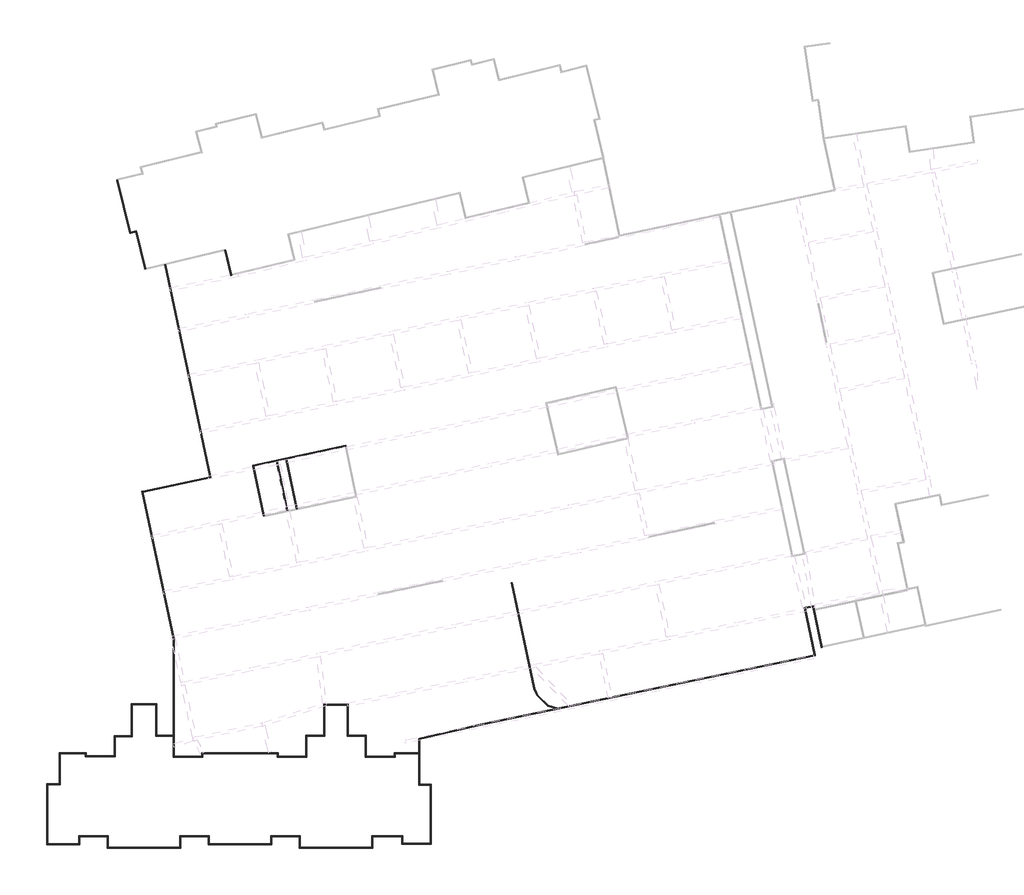
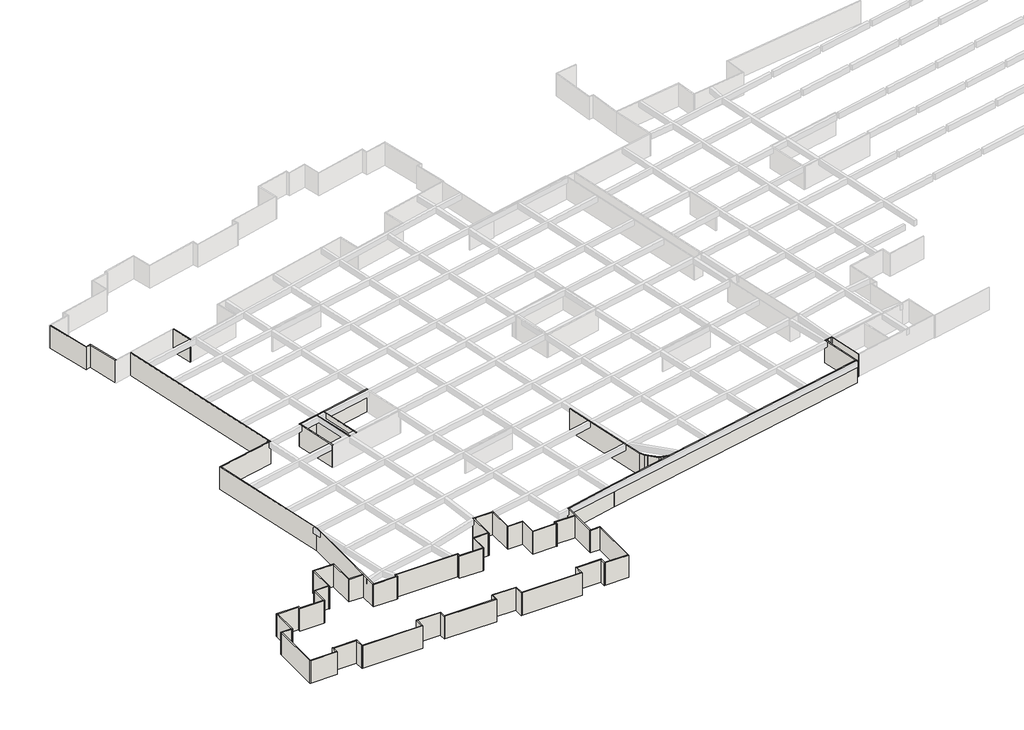
# One storey, part 1 of 14: 68 walls.
"""IFC4 building model written with IfcOpenShell, lengths in millimetres."""

from ifc_helpers import new_model, si_unit, origin, origin_with_axes, place, context, project, spatial, polyline, outline, extrude, faceted_brep, element, save

model = new_model("IFC4")

# Units and contexts
model_context = context("Model", 3, world=origin())
ifc_project = project(units=[si_unit("LENGTHUNIT", "METRE", prefix="MILLI")], contexts=[model_context])

# Site, building, storey
site = spatial("IfcSite", under=ifc_project)
building = spatial("IfcBuilding", under=site)
storey = spatial("IfcBuildingStorey", under=building, Name="户型图", Elevation=0.0)

# Walls
placement = place(None, origin())
element("IfcWall", 1, ObjectType="所有墙体", at=placement, inside=storey, context=model_context, shape_type="Brep", body=[
    faceted_brep([(-336633.0955644, -203222.3430669, 0.0), (-339553.0955247, -203222.3430669, 0.0), (-339553.0955247, -203222.3430669, 3300.0), (-336633.0955644, -203222.3430669, 3300.0), (-336633.0955644, -203342.3430669, 0.0), (-336633.0955644, -203342.3430669, 3300.0), (-336753.0955644, -203342.3430669, 3300.0), (-339433.0955247, -203342.3430669, 3300.0), (-339553.0955247, -203342.3430669, 3300.0), (-339553.0955247, -203342.3430669, 0.0), (-339433.0955247, -203342.3430669, 0.0), (-336753.0955644, -203342.3430669, 0.0)], [[[0, 1, 2, 3]], [[4, 5, 6, 7, 8, 9, 10, 11]], [[1, 0, 4, 11, 10, 9]], [[3, 2, 8, 7, 6, 5]], [[2, 1, 9, 8]], [[0, 3, 5, 4]]]),
])
element("IfcWall", 2, ObjectType="所有墙体", at=placement, inside=storey, context=model_context, shape_type="Brep", body=[
    faceted_brep([(-339553.0955247, -203342.3430669, 0.0), (-339553.0955247, -206922.3429831, 0.0), (-339553.0955247, -207042.3429831, 0.0), (-339553.0955247, -207042.3429831, 3300.0), (-339553.0955247, -206922.3429831, 3300.0), (-339553.0955247, -203342.3430669, 3300.0), (-339433.0955247, -203342.3430669, 0.0), (-339433.0955247, -203342.3430669, 3300.0), (-339433.0955247, -207042.3429831, 3300.0), (-339433.0955247, -207042.3429831, 0.0)], [[[0, 1, 2, 3, 4, 5]], [[6, 7, 8, 9]], [[2, 1, 0, 6, 9]], [[5, 4, 3, 8, 7]], [[0, 5, 7, 6]], [[3, 2, 9, 8]]]),
])
element("IfcWall", 3, ObjectType="所有墙体", at=placement, inside=storey, context=model_context, shape_type="Brep", body=[
    faceted_brep([(-339553.0955247, -206922.3429831, 0.0), (-341553.0955629, -206922.3429831, 0.0), (-341553.0955629, -206922.3429831, 3300.0), (-339553.0955247, -206922.3429831, 3300.0), (-339553.0955247, -207042.3429831, 0.0), (-339553.0955247, -207042.3429831, 3300.0), (-341433.0955629, -207042.3429831, 3300.0), (-341553.0955629, -207042.3429831, 3300.0), (-341553.0955629, -207042.3429831, 0.0), (-341433.0955629, -207042.3429831, 0.0)], [[[0, 1, 2, 3]], [[4, 5, 6, 7, 8, 9]], [[1, 0, 4, 9, 8]], [[3, 2, 7, 6, 5]], [[0, 3, 5, 4]], [[2, 1, 8, 7]]]),
])
element("IfcWall", 4, ObjectType="所有墙体", at=placement, inside=storey, context=model_context, shape_type="Brep", body=[
    faceted_brep([(-341553.0955629, -207042.3429831, 0.0), (-341553.0955629, -209222.3430662, 0.0), (-341553.0955629, -209342.3430662, 0.0), (-341553.0955629, -209342.3430662, 3300.0), (-341553.0955629, -209222.3430662, 3300.0), (-341553.0955629, -207042.3429831, 3300.0), (-341433.0955629, -207042.3429831, 0.0), (-341433.0955629, -207042.3429831, 3300.0), (-341433.0955629, -209342.3430662, 3300.0), (-341433.0955629, -209342.3430662, 0.0)], [[[0, 1, 2, 3, 4, 5]], [[6, 7, 8, 9]], [[2, 1, 0, 6, 9]], [[5, 4, 3, 8, 7]], [[0, 5, 7, 6]], [[3, 2, 9, 8]]]),
])
element("IfcWall", 5, ObjectType="所有墙体", at=placement, inside=storey, context=model_context, shape_type="Brep", body=[
    faceted_brep([(-341553.0955629, -209222.3430662, 0.0), (-344783.0955149, -209222.3430662, 0.0), (-344903.0955149, -209222.3430662, 0.0), (-344903.0955149, -209222.3430662, 3300.0), (-344783.0955149, -209222.3430662, 3300.0), (-341553.0955629, -209222.3430662, 3300.0), (-341553.0955629, -209342.3430662, 0.0), (-341553.0955629, -209342.3430662, 3300.0), (-344903.0955149, -209342.3430662, 3300.0), (-344903.0955149, -209342.3430662, 0.0)], [[[0, 1, 2, 3, 4, 5]], [[6, 7, 8, 9]], [[2, 1, 0, 6, 9]], [[5, 4, 3, 8, 7]], [[0, 5, 7, 6]], [[3, 2, 9, 8]]]),
])
element("IfcWall", 6, ObjectType="所有墙体", at=placement, inside=storey, context=model_context, shape_type="Brep", body=[
    faceted_brep([(-344783.0955149, -209222.3430662, 0.0), (-344783.0955149, -208872.3428754, 0.0), (-344783.0955149, -208872.3428754, 3300.0), (-344783.0955149, -209222.3430662, 3300.0), (-344903.0955149, -209222.3430662, 0.0), (-344903.0955149, -209222.3430662, 3300.0), (-344903.0955149, -208992.3428754, 3300.0), (-344903.0955149, -208872.3428754, 3300.0), (-344903.0955149, -208872.3428754, 0.0), (-344903.0955149, -208992.3428754, 0.0)], [[[0, 1, 2, 3]], [[4, 5, 6, 7, 8, 9]], [[1, 0, 4, 9, 8]], [[3, 2, 7, 6, 5]], [[0, 3, 5, 4]], [[2, 1, 8, 7]]]),
])
element("IfcWall", 7, ObjectType="所有墙体", at=placement, inside=storey, context=model_context, shape_type="Brep", body=[
    faceted_brep([(-344903.0955149, -208872.3428754, 0.0), (-347903.0955133, -208872.3428754, 0.0), (-347903.0955133, -208872.3428754, 3300.0), (-344903.0955149, -208872.3428754, 3300.0), (-344903.0955149, -208992.3428754, 0.0), (-344903.0955149, -208992.3428754, 3300.0), (-347783.0955133, -208992.3428754, 3300.0), (-347903.0955133, -208992.3428754, 3300.0), (-347903.0955133, -208992.3428754, 0.0), (-347783.0955133, -208992.3428754, 0.0)], [[[0, 1, 2, 3]], [[4, 5, 6, 7, 8, 9]], [[1, 0, 4, 9, 8]], [[3, 2, 7, 6, 5]], [[0, 3, 5, 4]], [[2, 1, 8, 7]]]),
])
element("IfcWall", 8, ObjectType="所有墙体", at=placement, inside=storey, context=model_context, shape_type="Brep", body=[
    faceted_brep([(-347903.0955133, -208992.3428754, 0.0), (-347903.0955133, -212472.3429639, 0.0), (-347903.0955133, -212592.3429639, 0.0), (-347903.0955133, -212592.3429639, 3300.0), (-347903.0955133, -212472.3429639, 3300.0), (-347903.0955133, -208992.3428754, 3300.0), (-347783.0955133, -208992.3428754, 0.0), (-347783.0955133, -208992.3428754, 3300.0), (-347783.0955133, -212592.3429639, 3300.0), (-347783.0955133, -212592.3429639, 0.0)], [[[0, 1, 2, 3, 4, 5]], [[6, 7, 8, 9]], [[2, 1, 0, 6, 9]], [[5, 4, 3, 8, 7]], [[0, 5, 7, 6]], [[3, 2, 9, 8]]]),
])
element("IfcWall", 9, ObjectType="所有墙体", at=placement, inside=storey, context=model_context, shape_type="Brep", body=[
    faceted_brep([(-347903.0955133, -212472.3429639, 0.0), (-349353.0955304, -212472.3429639, 0.0), (-349353.0955304, -212472.3429639, 3300.0), (-347903.0955133, -212472.3429639, 3300.0), (-347903.0955133, -212592.3429639, 0.0), (-347903.0955133, -212592.3429639, 3300.0), (-349233.0955304, -212592.3429639, 3300.0), (-349353.0955304, -212592.3429639, 3300.0), (-349353.0955304, -212592.3429639, 0.0), (-349233.0955304, -212592.3429639, 0.0)], [[[0, 1, 2, 3]], [[4, 5, 6, 7, 8, 9]], [[1, 0, 4, 9, 8]], [[3, 2, 7, 6, 5]], [[0, 3, 5, 4]], [[2, 1, 8, 7]]]),
])
element("IfcWall", 10, ObjectType="所有墙体", at=placement, inside=storey, context=model_context, shape_type="Brep", body=[
    faceted_brep([(-349353.0955304, -212592.3429639, 0.0), (-349353.0955304, -219492.3429639, 0.0), (-349353.0955304, -219492.3429639, 3300.0), (-349353.0955304, -212592.3429639, 3300.0), (-349233.0955304, -212592.3429639, 0.0), (-349233.0955304, -212592.3429639, 3300.0), (-349233.0955304, -219372.3429639, 3300.0), (-349233.0955304, -219492.3429639, 3300.0), (-349233.0955304, -219492.3429639, 0.0), (-349233.0955304, -219372.3429639, 0.0)], [[[0, 1, 2, 3]], [[4, 5, 6, 7, 8, 9]], [[1, 0, 4, 9, 8]], [[3, 2, 7, 6, 5]], [[0, 3, 5, 4]], [[2, 1, 8, 7]]]),
])
element("IfcWall", 11, ObjectType="所有墙体", at=placement, inside=storey, context=model_context, shape_type="Brep", body=[
    faceted_brep([(-349233.0955304, -219492.3429639, 0.0), (-345533.0955632, -219492.3429639, 0.0), (-345533.0955632, -219492.3429639, 3300.0), (-349233.0955304, -219492.3429639, 3300.0), (-349233.0955304, -219372.3429639, 0.0), (-349233.0955304, -219372.3429639, 3300.0), (-345653.0955632, -219372.3429639, 3300.0), (-345533.0955632, -219372.3429639, 3300.0), (-345533.0955632, -219372.3429639, 0.0), (-345653.0955632, -219372.3429639, 0.0)], [[[0, 1, 2, 3]], [[4, 5, 6, 7, 8, 9]], [[1, 0, 4, 9, 8]], [[3, 2, 7, 6, 5]], [[0, 3, 5, 4]], [[2, 1, 8, 7]]]),
])
element("IfcWall", 12, ObjectType="所有墙体", at=placement, inside=storey, context=model_context, shape_type="Brep", body=[
    faceted_brep([(-345533.0955632, -219372.3429639, 0.0), (-345533.0955632, -218592.3429692, 0.0), (-345533.0955632, -218472.3429692, 0.0), (-345533.0955632, -218472.3429692, 3300.0), (-345533.0955632, -218592.3429692, 3300.0), (-345533.0955632, -219372.3429639, 3300.0), (-345653.0955632, -219372.3429639, 0.0), (-345653.0955632, -219372.3429639, 3300.0), (-345653.0955632, -218472.3429692, 3300.0), (-345653.0955632, -218472.3429692, 0.0)], [[[0, 1, 2, 3, 4, 5]], [[6, 7, 8, 9]], [[2, 1, 0, 6, 9]], [[5, 4, 3, 8, 7]], [[0, 5, 7, 6]], [[3, 2, 9, 8]]]),
])
element("IfcWall", 13, ObjectType="所有墙体", at=placement, inside=storey, context=model_context, shape_type="Brep", body=[
    faceted_brep([(-345533.0955632, -218592.3429692, 0.0), (-342353.0955632, -218592.3429692, 0.0), (-342233.0955632, -218592.3429692, 0.0), (-342233.0955632, -218592.3429692, 3300.0), (-342353.0955632, -218592.3429692, 3300.0), (-345533.0955632, -218592.3429692, 3300.0), (-345533.0955632, -218472.3429692, 0.0), (-345533.0955632, -218472.3429692, 3300.0), (-342233.0955632, -218472.3429692, 3300.0), (-342233.0955632, -218472.3429692, 0.0)], [[[0, 1, 2, 3, 4, 5]], [[6, 7, 8, 9]], [[2, 1, 0, 6, 9]], [[5, 4, 3, 8, 7]], [[0, 5, 7, 6]], [[3, 2, 9, 8]]]),
])
element("IfcWall", 14, ObjectType="所有墙体", at=placement, inside=storey, context=model_context, shape_type="Brep", body=[
    faceted_brep([(-342353.0955632, -218592.3429692, 0.0), (-342353.0955632, -219892.3429766, 0.0), (-342353.0955632, -219892.3429766, 3300.0), (-342353.0955632, -218592.3429692, 3300.0), (-342233.0955632, -218592.3429692, 0.0), (-342233.0955632, -218592.3429692, 3300.0), (-342233.0955632, -219772.3429766, 3300.0), (-342233.0955632, -219892.3429766, 3300.0), (-342233.0955632, -219892.3429766, 0.0), (-342233.0955632, -219772.3429766, 0.0)], [[[0, 1, 2, 3]], [[4, 5, 6, 7, 8, 9]], [[1, 0, 4, 9, 8]], [[3, 2, 7, 6, 5]], [[0, 3, 5, 4]], [[2, 1, 8, 7]]]),
])
element("IfcWall", 15, ObjectType="所有墙体", at=placement, inside=storey, context=model_context, shape_type="Brep", body=[
    faceted_brep([(-342233.0955632, -219892.3429766, 0.0), (-333833.0955651, -219892.3429766, 0.0), (-333833.0955651, -219892.3429766, 3300.0), (-342233.0955632, -219892.3429766, 3300.0), (-342233.0955632, -219772.3429766, 0.0), (-342233.0955632, -219772.3429766, 3300.0), (-333953.0955651, -219772.3429766, 3300.0), (-333833.0955651, -219772.3429766, 3300.0), (-333833.0955651, -219772.3429766, 0.0), (-333953.0955651, -219772.3429766, 0.0)], [[[0, 1, 2, 3]], [[4, 5, 6, 7, 8, 9]], [[1, 0, 4, 9, 8]], [[3, 2, 7, 6, 5]], [[0, 3, 5, 4]], [[2, 1, 8, 7]]]),
])
element("IfcWall", 16, ObjectType="所有墙体", at=placement, inside=storey, context=model_context, shape_type="Brep", body=[
    faceted_brep([(-333833.0955651, -219772.3429766, 0.0), (-333833.0955651, -218592.3429692, 0.0), (-333833.0955651, -218472.3429692, 0.0), (-333833.0955651, -218472.3429692, 3300.0), (-333833.0955651, -218592.3429692, 3300.0), (-333833.0955651, -219772.3429766, 3300.0), (-333953.0955651, -219772.3429766, 0.0), (-333953.0955651, -219772.3429766, 3300.0), (-333953.0955651, -218472.3429692, 3300.0), (-333953.0955651, -218472.3429692, 0.0)], [[[0, 1, 2, 3, 4, 5]], [[6, 7, 8, 9]], [[2, 1, 0, 6, 9]], [[5, 4, 3, 8, 7]], [[0, 5, 7, 6]], [[3, 2, 9, 8]]]),
])
element("IfcWall", 17, ObjectType="所有墙体", at=placement, inside=storey, context=model_context, shape_type="Brep", body=[
    faceted_brep([(-333833.0955651, -218592.3429692, 0.0), (-330653.0955615, -218592.3429692, 0.0), (-330533.0955615, -218592.3429692, 0.0), (-330533.0955615, -218592.3429692, 3300.0), (-330653.0955615, -218592.3429692, 3300.0), (-333833.0955651, -218592.3429692, 3300.0), (-333833.0955651, -218472.3429692, 0.0), (-333833.0955651, -218472.3429692, 3300.0), (-330533.0955615, -218472.3429692, 3300.0), (-330533.0955615, -218472.3429692, 0.0)], [[[0, 1, 2, 3, 4, 5]], [[6, 7, 8, 9]], [[2, 1, 0, 6, 9]], [[5, 4, 3, 8, 7]], [[0, 5, 7, 6]], [[3, 2, 9, 8]]]),
])
element("IfcWall", 18, ObjectType="所有墙体", at=placement, inside=storey, context=model_context, shape_type="Brep", body=[
    faceted_brep([(-330653.0955615, -218592.3429692, 0.0), (-330653.0955615, -219492.3429639, 0.0), (-330653.0955615, -219492.3429639, 3300.0), (-330653.0955615, -218592.3429692, 3300.0), (-330533.0955615, -218592.3429692, 0.0), (-330533.0955615, -218592.3429692, 3300.0), (-330533.0955615, -219372.3429639, 3300.0), (-330533.0955615, -219492.3429639, 3300.0), (-330533.0955615, -219492.3429639, 0.0), (-330533.0955615, -219372.3429639, 0.0)], [[[0, 1, 2, 3]], [[4, 5, 6, 7, 8, 9]], [[1, 0, 4, 9, 8]], [[3, 2, 7, 6, 5]], [[0, 3, 5, 4]], [[2, 1, 8, 7]]]),
])
element("IfcWall", 19, ObjectType="所有墙体", at=placement, inside=storey, context=model_context, shape_type="Brep", body=[
    faceted_brep([(-330533.0955615, -219492.3429639, 0.0), (-323333.0955632, -219492.3429639, 0.0), (-323333.0955632, -219492.3429639, 3300.0), (-330533.0955615, -219492.3429639, 3300.0), (-330533.0955615, -219372.3429639, 0.0), (-330533.0955615, -219372.3429639, 3300.0), (-323453.0955632, -219372.3429639, 3300.0), (-323333.0955632, -219372.3429639, 3300.0), (-323333.0955632, -219372.3429639, 0.0), (-323453.0955632, -219372.3429639, 0.0)], [[[0, 1, 2, 3]], [[4, 5, 6, 7, 8, 9]], [[1, 0, 4, 9, 8]], [[3, 2, 7, 6, 5]], [[0, 3, 5, 4]], [[2, 1, 8, 7]]]),
])
element("IfcWall", 20, ObjectType="所有墙体", at=placement, inside=storey, context=model_context, shape_type="Brep", body=[
    faceted_brep([(-323333.0955632, -219372.3429639, 0.0), (-323333.0955632, -218592.3429692, 0.0), (-323333.0955632, -218472.3429692, 0.0), (-323333.0955632, -218472.3429692, 3300.0), (-323333.0955632, -218592.3429692, 3300.0), (-323333.0955632, -219372.3429639, 3300.0), (-323453.0955632, -219372.3429639, 0.0), (-323453.0955632, -219372.3429639, 3300.0), (-323453.0955632, -218472.3429692, 3300.0), (-323453.0955632, -218472.3429692, 0.0)], [[[0, 1, 2, 3, 4, 5]], [[6, 7, 8, 9]], [[2, 1, 0, 6, 9]], [[5, 4, 3, 8, 7]], [[0, 5, 7, 6]], [[3, 2, 9, 8]]]),
])
element("IfcWall", 21, ObjectType="所有墙体", at=placement, inside=storey, context=model_context, shape_type="Brep", body=[
    faceted_brep([(-323333.0955632, -218592.3429692, 0.0), (-320153.095561, -218592.3429692, 0.0), (-320033.095561, -218592.3429692, 0.0), (-320033.095561, -218592.3429692, 3300.0), (-320153.095561, -218592.3429692, 3300.0), (-323333.0955632, -218592.3429692, 3300.0), (-323333.0955632, -218472.3429692, 0.0), (-323333.0955632, -218472.3429692, 3300.0), (-320033.095561, -218472.3429692, 3300.0), (-320033.095561, -218472.3429692, 0.0)], [[[0, 1, 2, 3, 4, 5]], [[6, 7, 8, 9]], [[2, 1, 0, 6, 9]], [[5, 4, 3, 8, 7]], [[0, 5, 7, 6]], [[3, 2, 9, 8]]]),
])
element("IfcWall", 22, ObjectType="所有墙体", at=placement, inside=storey, context=model_context, shape_type="Brep", body=[
    faceted_brep([(-320153.095561, -218592.3429692, 0.0), (-320153.095561, -219892.3429766, 0.0), (-320153.095561, -219892.3429766, 3300.0), (-320153.095561, -218592.3429692, 3300.0), (-320033.095561, -218592.3429692, 0.0), (-320033.095561, -218592.3429692, 3300.0), (-320033.095561, -219772.3429766, 3300.0), (-320033.095561, -219892.3429766, 3300.0), (-320033.095561, -219892.3429766, 0.0), (-320033.095561, -219772.3429766, 0.0)], [[[0, 1, 2, 3]], [[4, 5, 6, 7, 8, 9]], [[1, 0, 4, 9, 8]], [[3, 2, 7, 6, 5]], [[0, 3, 5, 4]], [[2, 1, 8, 7]]]),
])
element("IfcWall", 23, ObjectType="所有墙体", at=placement, inside=storey, context=model_context, shape_type="Brep", body=[
    faceted_brep([(-320033.095561, -219892.3429766, 0.0), (-311633.0955651, -219892.3429766, 0.0), (-311633.0955651, -219892.3429766, 3300.0), (-320033.095561, -219892.3429766, 3300.0), (-320033.095561, -219772.3429766, 0.0), (-320033.095561, -219772.3429766, 3300.0), (-311753.0955651, -219772.3429766, 3300.0), (-311633.0955651, -219772.3429766, 3300.0), (-311633.0955651, -219772.3429766, 0.0), (-311753.0955651, -219772.3429766, 0.0)], [[[0, 1, 2, 3]], [[4, 5, 6, 7, 8, 9]], [[1, 0, 4, 9, 8]], [[3, 2, 7, 6, 5]], [[0, 3, 5, 4]], [[2, 1, 8, 7]]]),
])
element("IfcWall", 24, ObjectType="所有墙体", at=placement, inside=storey, context=model_context, shape_type="Brep", body=[
    faceted_brep([(-311633.0955651, -219772.3429766, 0.0), (-311633.0955651, -218592.3429692, 0.0), (-311633.0955651, -218472.3429692, 0.0), (-311633.0955651, -218472.3429692, 3300.0), (-311633.0955651, -218592.3429692, 3300.0), (-311633.0955651, -219772.3429766, 3300.0), (-311753.0955651, -219772.3429766, 0.0), (-311753.0955651, -219772.3429766, 3300.0), (-311753.0955651, -218472.3429692, 3300.0), (-311753.0955651, -218472.3429692, 0.0)], [[[0, 1, 2, 3, 4, 5]], [[6, 7, 8, 9]], [[2, 1, 0, 6, 9]], [[5, 4, 3, 8, 7]], [[0, 5, 7, 6]], [[3, 2, 9, 8]]]),
])
element("IfcWall", 25, ObjectType="所有墙体", at=placement, inside=storey, context=model_context, shape_type="Brep", body=[
    faceted_brep([(-311633.0955651, -218592.3429692, 0.0), (-308303.095558, -218592.3429692, 0.0), (-308183.095558, -218592.3429692, 0.0), (-308183.095558, -218592.3429692, 3300.0), (-308303.095558, -218592.3429692, 3300.0), (-311633.0955651, -218592.3429692, 3300.0), (-311633.0955651, -218472.3429692, 0.0), (-311633.0955651, -218472.3429692, 3300.0), (-308183.095558, -218472.3429692, 3300.0), (-308183.095558, -218472.3429692, 0.0)], [[[0, 1, 2, 3, 4, 5]], [[6, 7, 8, 9]], [[2, 1, 0, 6, 9]], [[5, 4, 3, 8, 7]], [[0, 5, 7, 6]], [[3, 2, 9, 8]]]),
])
element("IfcWall", 26, ObjectType="所有墙体", at=placement, inside=storey, context=model_context, shape_type="Brep", body=[
    faceted_brep([(-308303.095558, -218592.3429692, 0.0), (-308303.095558, -219442.3430493, 0.0), (-308303.095558, -219442.3430493, 3300.0), (-308303.095558, -218592.3429692, 3300.0), (-308183.095558, -218592.3429692, 0.0), (-308183.095558, -218592.3429692, 3300.0), (-308183.095558, -219322.3430493, 3300.0), (-308183.095558, -219442.3430493, 3300.0), (-308183.095558, -219442.3430493, 0.0), (-308183.095558, -219322.3430493, 0.0)], [[[0, 1, 2, 3]], [[4, 5, 6, 7, 8, 9]], [[1, 0, 4, 9, 8]], [[3, 2, 7, 6, 5]], [[0, 3, 5, 4]], [[2, 1, 8, 7]]]),
])
element("IfcWall", 27, ObjectType="所有墙体", at=placement, inside=storey, context=model_context, shape_type="Brep", body=[
    faceted_brep([(-308183.095558, -219442.3430493, 0.0), (-304883.0955621, -219442.3430493, 0.0), (-304883.0955621, -219442.3430493, 3300.0), (-308183.095558, -219442.3430493, 3300.0), (-308183.095558, -219322.3430493, 0.0), (-308183.095558, -219322.3430493, 3300.0), (-305003.0955621, -219322.3430493, 3300.0), (-304883.0955621, -219322.3430493, 3300.0), (-304883.0955621, -219322.3430493, 0.0), (-305003.0955621, -219322.3430493, 0.0)], [[[0, 1, 2, 3]], [[4, 5, 6, 7, 8, 9]], [[1, 0, 4, 9, 8]], [[3, 2, 7, 6, 5]], [[0, 3, 5, 4]], [[2, 1, 8, 7]]]),
])
element("IfcWall", 28, ObjectType="所有墙体", at=placement, inside=storey, context=model_context, shape_type="Brep", body=[
    faceted_brep([(-304883.0955621, -219322.3430493, 0.0), (-304883.0955621, -212522.3430493, 0.0), (-304883.0955621, -212522.3430493, 3300.0), (-304883.0955621, -219322.3430493, 3300.0), (-305003.0955621, -219322.3430493, 0.0), (-305003.0955621, -219322.3430493, 3300.0), (-305003.0955621, -212642.3430493, 3300.0), (-305003.0955621, -212522.3430493, 3300.0), (-305003.0955621, -212522.3430493, 0.0), (-305003.0955621, -212642.3430493, 0.0)], [[[0, 1, 2, 3]], [[4, 5, 6, 7, 8, 9]], [[1, 0, 4, 9, 8]], [[3, 2, 7, 6, 5]], [[0, 3, 5, 4]], [[2, 1, 8, 7]]]),
])
element("IfcWall", 29, ObjectType="所有墙体", at=placement, inside=storey, context=model_context, shape_type="Brep", body=[
    faceted_brep([(-305003.0955621, -212522.3430493, 0.0), (-306233.0955314, -212522.3430493, 0.0), (-306353.0955314, -212522.3430493, 0.0), (-306353.0955314, -212522.3430493, 3300.0), (-306233.0955314, -212522.3430493, 3300.0), (-305003.0955621, -212522.3430493, 3300.0), (-305003.0955621, -212642.3430493, 0.0), (-305003.0955621, -212642.3430493, 3300.0), (-306353.0955314, -212642.3430493, 3300.0), (-306353.0955314, -212642.3430493, 0.0)], [[[0, 1, 2, 3, 4, 5]], [[6, 7, 8, 9]], [[2, 1, 0, 6, 9]], [[5, 4, 3, 8, 7]], [[0, 5, 7, 6]], [[3, 2, 9, 8]]]),
])
element("IfcWall", 30, ObjectType="所有墙体", at=placement, inside=storey, context=model_context, shape_type="Brep", body=[
    faceted_brep([(-306233.0955314, -212522.3430493, 0.0), (-306233.0955314, -207340.9733644, 0.0), (-306233.0955314, -207217.8168715, 0.0), (-306233.0955314, -207217.8168715, 3300.0), (-306233.0955314, -207340.9733644, 3300.0), (-306233.0955314, -212522.3430493, 3300.0), (-306353.0955314, -212522.3430493, 0.0), (-306353.0955314, -212522.3430493, 3300.0), (-306353.0955314, -208992.3430586, 3300.0), (-306353.0955314, -208872.3430586, 3300.0), (-306353.0955314, -207245.5210544, 3300.0), (-306353.0955314, -207245.5210544, 0.0), (-306353.0955314, -208872.3430586, 0.0), (-306353.0955314, -208992.3430586, 0.0)], [[[0, 1, 2, 3, 4, 5]], [[6, 7, 8, 9, 10, 11, 12, 13]], [[2, 1, 0, 6, 13, 12, 11]], [[5, 4, 3, 10, 9, 8, 7]], [[0, 5, 7, 6]], [[3, 2, 11, 10]]]),
])
element("IfcWall", 31, ObjectType="所有墙体", at=placement, inside=storey, context=model_context, shape_type="Brep", body=[
    faceted_brep([(-306353.0955314, -208872.3430586, 0.0), (-309203.0955142, -208872.3430586, 0.0), (-309203.0955142, -208872.3430586, 3300.0), (-306353.0955314, -208872.3430586, 3300.0), (-306353.0955314, -208992.3430586, 0.0), (-306353.0955314, -208992.3430586, 3300.0), (-309083.0955142, -208992.3430586, 3300.0), (-309203.0955142, -208992.3430586, 3300.0), (-309203.0955142, -208992.3430586, 0.0), (-309083.0955142, -208992.3430586, 0.0)], [[[0, 1, 2, 3]], [[4, 5, 6, 7, 8, 9]], [[1, 0, 4, 9, 8]], [[3, 2, 7, 6, 5]], [[0, 3, 5, 4]], [[2, 1, 8, 7]]]),
])
element("IfcWall", 32, ObjectType="所有墙体", at=placement, inside=storey, context=model_context, shape_type="Brep", body=[
    faceted_brep([(-309203.0955142, -208992.3430586, 0.0), (-309203.0955142, -209272.3430424, 0.0), (-309203.0955142, -209392.3430424, 0.0), (-309203.0955142, -209392.3430424, 3300.0), (-309203.0955142, -209272.3430424, 3300.0), (-309203.0955142, -208992.3430586, 3300.0), (-309083.0955142, -208992.3430586, 0.0), (-309083.0955142, -208992.3430586, 3300.0), (-309083.0955142, -209392.3430424, 3300.0), (-309083.0955142, -209392.3430424, 0.0)], [[[0, 1, 2, 3, 4, 5]], [[6, 7, 8, 9]], [[2, 1, 0, 6, 9]], [[5, 4, 3, 8, 7]], [[0, 5, 7, 6]], [[3, 2, 9, 8]]]),
])
element("IfcWall", 33, ObjectType="所有墙体", at=placement, inside=storey, context=model_context, shape_type="Brep", body=[
    faceted_brep([(-309203.0955142, -209272.3430424, 0.0), (-312383.0955095, -209272.3430424, 0.0), (-312503.0955095, -209272.3430424, 0.0), (-312503.0955095, -209272.3430424, 3300.0), (-312383.0955095, -209272.3430424, 3300.0), (-309203.0955142, -209272.3430424, 3300.0), (-309203.0955142, -209392.3430424, 0.0), (-309203.0955142, -209392.3430424, 3300.0), (-312503.0955095, -209392.3430424, 3300.0), (-312503.0955095, -209392.3430424, 0.0)], [[[0, 1, 2, 3, 4, 5]], [[6, 7, 8, 9]], [[2, 1, 0, 6, 9]], [[5, 4, 3, 8, 7]], [[0, 5, 7, 6]], [[3, 2, 9, 8]]]),
])
element("IfcWall", 34, ObjectType="所有墙体", at=placement, inside=storey, context=model_context, shape_type="Brep", body=[
    faceted_brep([(-312383.0955095, -209272.3430424, 0.0), (-312383.0955095, -206872.3430284, 0.0), (-312383.0955095, -206872.3430284, 3300.0), (-312383.0955095, -209272.3430424, 3300.0), (-312503.0955095, -209272.3430424, 0.0), (-312503.0955095, -209272.3430424, 3300.0), (-312503.0955095, -206992.3430284, 3300.0), (-312503.0955095, -206872.3430284, 3300.0), (-312503.0955095, -206872.3430284, 0.0), (-312503.0955095, -206992.3430284, 0.0)], [[[0, 1, 2, 3]], [[4, 5, 6, 7, 8, 9]], [[1, 0, 4, 9, 8]], [[3, 2, 7, 6, 5]], [[0, 3, 5, 4]], [[2, 1, 8, 7]]]),
])
element("IfcWall", 35, ObjectType="所有墙体", at=placement, inside=storey, context=model_context, shape_type="Brep", body=[
    faceted_brep([(-312503.0955095, -206872.3430284, 0.0), (-314483.0955038, -206872.3430284, 0.0), (-314603.0955038, -206872.3430284, 0.0), (-314603.0955038, -206872.3430284, 3300.0), (-314483.0955038, -206872.3430284, 3300.0), (-312503.0955095, -206872.3430284, 3300.0), (-312503.0955095, -206992.3430284, 0.0), (-312503.0955095, -206992.3430284, 3300.0), (-314603.0955038, -206992.3430284, 3300.0), (-314603.0955038, -206992.3430284, 0.0)], [[[0, 1, 2, 3, 4, 5]], [[6, 7, 8, 9]], [[2, 1, 0, 6, 9]], [[5, 4, 3, 8, 7]], [[0, 5, 7, 6]], [[3, 2, 9, 8]]]),
])
element("IfcWall", 36, ObjectType="所有墙体", at=placement, inside=storey, context=model_context, shape_type="Brep", body=[
    faceted_brep([(-314483.0955038, -206872.3430284, 0.0), (-314483.0955038, -203272.343013, 0.0), (-314483.0955038, -203272.343013, 3300.0), (-314483.0955038, -206872.3430284, 3300.0), (-314603.0955038, -206872.3430284, 0.0), (-314603.0955038, -206872.3430284, 3300.0), (-314603.0955038, -203392.343013, 3300.0), (-314603.0955038, -203272.343013, 3300.0), (-314603.0955038, -203272.343013, 0.0), (-314603.0955038, -203392.343013, 0.0)], [[[0, 1, 2, 3]], [[4, 5, 6, 7, 8, 9]], [[1, 0, 4, 9, 8]], [[3, 2, 7, 6, 5]], [[0, 3, 5, 4]], [[2, 1, 8, 7]]]),
])
element("IfcWall", 37, ObjectType="所有墙体", at=placement, inside=storey, context=model_context, shape_type="Brep", body=[
    faceted_brep([(-314603.0955038, -203272.343013, 0.0), (-317303.0954912, -203272.343013, 0.0), (-317303.0954912, -203272.343013, 3300.0), (-314603.0955038, -203272.343013, 3300.0), (-314603.0955038, -203392.343013, 0.0), (-314603.0955038, -203392.343013, 3300.0), (-317183.0954912, -203392.343013, 3300.0), (-317303.0954912, -203392.343013, 3300.0), (-317303.0954912, -203392.343013, 0.0), (-317183.0954912, -203392.343013, 0.0)], [[[0, 1, 2, 3]], [[4, 5, 6, 7, 8, 9]], [[1, 0, 4, 9, 8]], [[3, 2, 7, 6, 5]], [[0, 3, 5, 4]], [[2, 1, 8, 7]]]),
])
element("IfcWall", 38, ObjectType="所有墙体", at=placement, inside=storey, context=model_context, shape_type="Brep", body=[
    faceted_brep([(-317303.0954912, -203392.343013, 0.0), (-317303.0954912, -206872.3430284, 0.0), (-317303.0954912, -206992.3430284, 0.0), (-317303.0954912, -206992.3430284, 3300.0), (-317303.0954912, -206872.3430284, 3300.0), (-317303.0954912, -203392.343013, 3300.0), (-317183.0954912, -203392.343013, 0.0), (-317183.0954912, -203392.343013, 3300.0), (-317183.0954912, -206992.3430284, 3300.0), (-317183.0954912, -206992.3430284, 0.0)], [[[0, 1, 2, 3, 4, 5]], [[6, 7, 8, 9]], [[2, 1, 0, 6, 9]], [[5, 4, 3, 8, 7]], [[0, 5, 7, 6]], [[3, 2, 9, 8]]]),
])
element("IfcWall", 39, ObjectType="所有墙体", at=placement, inside=storey, context=model_context, shape_type="Brep", body=[
    faceted_brep([(-317303.0954912, -206872.3430284, 0.0), (-319403.0955072, -206872.3430284, 0.0), (-319403.0955072, -206872.3430284, 3300.0), (-317303.0954912, -206872.3430284, 3300.0), (-317303.0954912, -206992.3430284, 0.0), (-317303.0954912, -206992.3430284, 3300.0), (-319283.0955072, -206992.3430284, 3300.0), (-319403.0955072, -206992.3430284, 3300.0), (-319403.0955072, -206992.3430284, 0.0), (-319283.0955072, -206992.3430284, 0.0)], [[[0, 1, 2, 3]], [[4, 5, 6, 7, 8, 9]], [[1, 0, 4, 9, 8]], [[3, 2, 7, 6, 5]], [[0, 3, 5, 4]], [[2, 1, 8, 7]]]),
])
element("IfcWall", 40, ObjectType="所有墙体", at=placement, inside=storey, context=model_context, shape_type="Brep", body=[
    faceted_brep([(-319403.0955072, -206992.3430284, 0.0), (-319403.0955072, -209272.3430424, 0.0), (-319403.0955072, -209392.3430424, 0.0), (-319403.0955072, -209392.3430424, 3300.0), (-319403.0955072, -209272.3430424, 3300.0), (-319403.0955072, -206992.3430284, 3300.0), (-319283.0955072, -206992.3430284, 0.0), (-319283.0955072, -206992.3430284, 3300.0), (-319283.0955072, -209392.3430424, 3300.0), (-319283.0955072, -209392.3430424, 0.0)], [[[0, 1, 2, 3, 4, 5]], [[6, 7, 8, 9]], [[2, 1, 0, 6, 9]], [[5, 4, 3, 8, 7]], [[0, 5, 7, 6]], [[3, 2, 9, 8]]]),
])
element("IfcWall", 41, ObjectType="所有墙体", at=placement, inside=storey, context=model_context, shape_type="Brep", body=[
    faceted_brep([(-319403.0955072, -209272.3430424, 0.0), (-322583.0955166, -209272.3430424, 0.0), (-322703.0955166, -209272.3430424, 0.0), (-322703.0955166, -209272.3430424, 3300.0), (-322583.0955166, -209272.3430424, 3300.0), (-319403.0955072, -209272.3430424, 3300.0), (-319403.0955072, -209392.3430424, 0.0), (-319403.0955072, -209392.3430424, 3300.0), (-322703.0955166, -209392.3430424, 3300.0), (-322703.0955166, -209392.3430424, 0.0)], [[[0, 1, 2, 3, 4, 5]], [[6, 7, 8, 9]], [[2, 1, 0, 6, 9]], [[5, 4, 3, 8, 7]], [[0, 5, 7, 6]], [[3, 2, 9, 8]]]),
])
element("IfcWall", 42, ObjectType="所有墙体", at=placement, inside=storey, context=model_context, shape_type="Brep", body=[
    faceted_brep([(-322583.0955166, -209272.3430424, 0.0), (-322583.0955166, -208872.3430586, 0.0), (-322583.0955166, -208872.3430586, 3300.0), (-322583.0955166, -209272.3430424, 3300.0), (-322703.0955166, -209272.3430424, 0.0), (-322703.0955166, -209272.3430424, 3300.0), (-322703.0955166, -208992.3430586, 3300.0), (-322703.0955166, -208872.3430586, 3300.0), (-322703.0955166, -208872.3430586, 0.0), (-322703.0955166, -208992.3430586, 0.0)], [[[0, 1, 2, 3]], [[4, 5, 6, 7, 8, 9]], [[1, 0, 4, 9, 8]], [[3, 2, 7, 6, 5]], [[0, 3, 5, 4]], [[2, 1, 8, 7]]]),
])
element("IfcWall", 43, ObjectType="所有墙体", at=placement, inside=storey, context=model_context, shape_type="Brep", body=[
    faceted_brep([(-322703.0955166, -208872.3430586, 0.0), (-331403.0955142, -208872.3430586, 0.0), (-331403.0955142, -208872.3430586, 3300.0), (-322703.0955166, -208872.3430586, 3300.0), (-322703.0955166, -208992.3430586, 0.0), (-322703.0955166, -208992.3430586, 3300.0), (-331283.0955142, -208992.3430586, 3300.0), (-331403.0955142, -208992.3430586, 3300.0), (-331403.0955142, -208992.3430586, 0.0), (-331283.0955142, -208992.3430586, 0.0)], [[[0, 1, 2, 3]], [[4, 5, 6, 7, 8, 9]], [[1, 0, 4, 9, 8]], [[3, 2, 7, 6, 5]], [[0, 3, 5, 4]], [[2, 1, 8, 7]]]),
])
element("IfcWall", 44, ObjectType="所有墙体", at=placement, inside=storey, context=model_context, shape_type="Brep", body=[
    faceted_brep([(-331403.0955142, -208992.3430586, 0.0), (-331403.0955142, -209272.3430424, 0.0), (-331403.0955142, -209392.3430424, 0.0), (-331403.0955142, -209392.3430424, 3300.0), (-331403.0955142, -209272.3430424, 3300.0), (-331403.0955142, -208992.3430586, 3300.0), (-331283.0955142, -208992.3430586, 0.0), (-331283.0955142, -208992.3430586, 3300.0), (-331283.0955142, -209392.3430424, 3300.0), (-331283.0955142, -209392.3430424, 0.0)], [[[0, 1, 2, 3, 4, 5]], [[6, 7, 8, 9]], [[2, 1, 0, 6, 9]], [[5, 4, 3, 8, 7]], [[0, 5, 7, 6]], [[3, 2, 9, 8]]]),
])
element("IfcWall", 45, ObjectType="所有墙体", at=placement, inside=storey, context=model_context, shape_type="Brep", body=[
    faceted_brep([(-331403.0955142, -209272.3430424, 0.0), (-334583.0955129, -209272.3430424, 0.0), (-334703.0955129, -209272.3430424, 0.0), (-334703.0955129, -209272.3430424, 3300.0), (-334583.0955129, -209272.3430424, 3300.0), (-331403.0955142, -209272.3430424, 3300.0), (-331403.0955142, -209392.3430424, 0.0), (-331403.0955142, -209392.3430424, 3300.0), (-334703.0955129, -209392.3430424, 3300.0), (-334703.0955129, -209392.3430424, 0.0)], [[[0, 1, 2, 3, 4, 5]], [[6, 7, 8, 9]], [[2, 1, 0, 6, 9]], [[5, 4, 3, 8, 7]], [[0, 5, 7, 6]], [[3, 2, 9, 8]]]),
])
element("IfcWall", 46, ObjectType="所有墙体", at=placement, inside=storey, context=model_context, shape_type="Brep", body=[
    faceted_brep([(-334583.0955129, -209272.3430424, 0.0), (-334583.0955129, -195726.0367743, 0.0), (-334583.0955129, -195726.0367743, 3300.0), (-334583.0955129, -209272.3430424, 3300.0), (-334703.0955129, -209272.3430424, 0.0), (-334703.0955129, -209272.3430424, 3300.0), (-334703.0955129, -206992.3430284, 3300.0), (-334703.0955129, -206872.3430284, 3300.0), (-334703.0955129, -195738.6492825, 3300.0), (-334703.0955129, -195738.6492825, 0.0), (-334703.0955129, -206872.3430284, 0.0), (-334703.0955129, -206992.3430284, 0.0)], [[[0, 1, 2, 3]], [[4, 5, 6, 7, 8, 9, 10, 11]], [[1, 0, 4, 11, 10, 9]], [[3, 2, 8, 7, 6, 5]], [[0, 3, 5, 4]], [[2, 1, 9, 8]]]),
])
element("IfcWall", 47, ObjectType="所有墙体", at=placement, inside=storey, context=model_context, shape_type="Brep", body=[
    faceted_brep([(-334703.0955129, -206872.3430284, 0.0), (-336633.0955644, -206872.3430284, 0.0), (-336753.0955644, -206872.3430284, 0.0), (-336753.0955644, -206872.3430284, 3300.0), (-336633.0955644, -206872.3430284, 3300.0), (-334703.0955129, -206872.3430284, 3300.0), (-334703.0955129, -206992.3430284, 0.0), (-334703.0955129, -206992.3430284, 3300.0), (-336753.0955644, -206992.3430284, 3300.0), (-336753.0955644, -206992.3430284, 0.0)], [[[0, 1, 2, 3, 4, 5]], [[6, 7, 8, 9]], [[2, 1, 0, 6, 9]], [[5, 4, 3, 8, 7]], [[0, 5, 7, 6]], [[3, 2, 9, 8]]]),
])
element("IfcWall", 48, ObjectType="所有墙体", at=placement, inside=storey, context=model_context, shape_type="SweptSolid", body=[
    extrude(outline(polyline([(-336633.0955644, -203342.3430669), (-336633.0955644, -206872.3430284), (-336753.0955644, -206872.3430284), (-336753.0955644, -203342.3430669), (-336633.0955644, -203342.3430669)])), origin_with_axes(), (0.0, 0.0, 1.0), 3300.0),
])
element("IfcWall", 49, ObjectType="所有墙体", at=placement, inside=storey, context=model_context, shape_type="Brep", body=[
    faceted_brep([(-328767.5797313, -150832.3104387, 0.0), (-328059.9452667, -153747.6583448, 0.0), (-328059.9452667, -153747.6583448, 3300.0), (-328767.5797313, -150832.3104387, 3300.0), (-328650.9658147, -150804.0050601, 0.0), (-328650.9658147, -150804.0050601, 3300.0), (-327971.6367288, -153602.7390496, 3300.0), (-327943.3313501, -153719.3529662, 3300.0), (-327943.3313501, -153719.3529662, 0.0), (-327971.6367288, -153602.7390496, 0.0)], [[[0, 1, 2, 3]], [[4, 5, 6, 7, 8, 9]], [[1, 0, 4, 9, 8]], [[3, 2, 7, 6, 5]], [[0, 3, 5, 4]], [[2, 1, 8, 7]]]),
])
element("IfcWall", 50, ObjectType="所有墙体", at=placement, inside=storey, context=model_context, shape_type="Brep", body=[
    faceted_brep([(-341227.2467241, -142743.015133, 0.0), (-339741.2143432, -148865.245757, 0.0), (-339741.2143432, -148865.245757, 3300.0), (-341227.2467241, -142743.015133, 3300.0), (-341110.6328075, -142714.7097543, 0.0), (-341110.6328075, -142714.7097543, 3300.0), (-339652.9058053, -148720.3264618, 3300.0), (-339624.6004266, -148836.9403784, 3300.0), (-339624.6004266, -148836.9403784, 0.0), (-339652.9058053, -148720.3264618, 0.0)], [[[0, 1, 2, 3]], [[4, 5, 6, 7, 8, 9]], [[1, 0, 4, 9, 8]], [[3, 2, 7, 6, 5]], [[0, 3, 5, 4]], [[2, 1, 8, 7]]]),
])
element("IfcWall", 51, ObjectType="所有墙体", at=placement, inside=storey, context=model_context, shape_type="Brep", body=[
    faceted_brep([(-339624.6004266, -148836.9403784, 0.0), (-339060.9664969, -148700.1310482, 0.0), (-338944.3525803, -148671.8256696, 0.0), (-338944.3525803, -148671.8256696, 3300.0), (-339060.9664969, -148700.1310482, 3300.0), (-339624.6004266, -148836.9403784, 3300.0), (-339652.9058053, -148720.3264618, 0.0), (-339652.9058053, -148720.3264618, 3300.0), (-338972.657959, -148555.211753, 3300.0), (-338972.657959, -148555.211753, 0.0)], [[[0, 1, 2, 3, 4, 5]], [[6, 7, 8, 9]], [[2, 1, 0, 6, 9]], [[5, 4, 3, 8, 7]], [[0, 5, 7, 6]], [[3, 2, 9, 8]]]),
])
element("IfcWall", 52, ObjectType="所有墙体", at=placement, inside=storey, context=model_context, shape_type="SweptSolid", body=[
    extrude(outline(polyline([(-338027.8201762, -152956.5390008), (-339060.9664969, -148700.1310482), (-338944.3525803, -148671.8256696), (-337911.2062596, -152928.2336221), (-338027.8201762, -152956.5390008)])), origin_with_axes(), (0.0, 0.0, 1.0), 3300.0),
])
element("IfcWall", 53, ObjectType="所有墙体", at=placement, inside=storey, context=model_context, shape_type="Brep", body=[
    faceted_brep([(-334583.0955129, -195726.0367743, 0.0), (-338189.5953757, -178758.7889302, 0.0), (-338214.5447786, -178641.4112182, 0.0), (-338214.5447786, -178641.4112182, 3300.0), (-338189.5953757, -178758.7889302, 3300.0), (-334583.0955129, -195726.0367743, 3300.0), (-334703.0955129, -195738.6492825, 0.0), (-334703.0955129, -195738.6492825, 3300.0), (-338331.9224906, -178666.3606211, 3300.0), (-338331.9224906, -178666.3606211, 0.0)], [[[0, 1, 2, 3, 4, 5]], [[6, 7, 8, 9]], [[2, 1, 0, 6, 9]], [[5, 4, 3, 8, 7]], [[0, 5, 7, 6]], [[3, 2, 9, 8]]]),
])
element("IfcWall", 54, ObjectType="所有墙体", at=placement, inside=storey, context=model_context, shape_type="Brep", body=[
    faceted_brep([(-338189.5953757, -178758.7889302, 0.0), (-330364.4145698, -177095.4954037, 0.0), (-330364.4145698, -177095.4954037, 3300.0), (-338189.5953757, -178758.7889302, 3300.0), (-338214.5447786, -178641.4112182, 0.0), (-338214.5447786, -178641.4112182, 3300.0), (-330506.7416848, -177003.0670945, 3300.0), (-330389.3639727, -176978.1176916, 3300.0), (-330389.3639727, -176978.1176916, 0.0), (-330506.7416848, -177003.0670945, 0.0)], [[[0, 1, 2, 3]], [[4, 5, 6, 7, 8, 9]], [[1, 0, 4, 9, 8]], [[3, 2, 7, 6, 5]], [[0, 3, 5, 4]], [[2, 1, 8, 7]]]),
])
element("IfcWall", 55, ObjectType="所有墙体", at=placement, inside=storey, context=model_context, shape_type="SweptSolid", body=[
    extrude(outline(polyline([(-335594.5985969, -152489.4141517), (-330389.3639727, -176978.1176916), (-330506.7416848, -177003.0670945), (-335711.2604986, -152517.7311777), (-335594.5985969, -152489.4141517)])), origin_with_axes(), (0.0, 0.0, 1.0), 3300.0),
])
element("IfcWall", 56, ObjectType="所有墙体", at=placement, inside=storey, context=model_context, shape_type="SweptSolid", body=[
    extrude(outline(polyline([(-298972.4762269, -205664.7273191), (-306233.0955314, -207340.9733644), (-306233.0955314, -207217.8168715), (-298998.1638642, -205547.5012846), (-298972.4762269, -205664.7273191)])), origin_with_axes(), (0.0, 0.0, 1.0), 3300.0),
])
element("IfcWall", 57, ObjectType="所有墙体", at=placement, inside=storey, context=model_context, shape_type="Brep", body=[
    faceted_brep([(-298972.4762269, -205664.7273191, 0.0), (-260531.5751567, -197690.2628613, 0.0), (-260531.5751567, -197690.2628613, 3300.0), (-298972.4762269, -205664.7273191, 3300.0), (-298998.1638642, -205547.5012846, 0.0), (-298998.1638642, -205547.5012846, 3300.0), (-290471.2563264, -203778.6166018, 3300.0), (-290209.9310515, -203724.4053565, 3300.0), (-260673.4482841, -197597.139203, 3300.0), (-260555.9498912, -197572.7644685, 3300.0), (-260555.9498912, -197572.7644685, 0.0), (-260673.4482841, -197597.139203, 0.0), (-290209.9310515, -203724.4053565, 0.0), (-290471.2563264, -203778.6166018, 0.0)], [[[0, 1, 2, 3]], [[4, 5, 6, 7, 8, 9, 10, 11, 12, 13]], [[1, 0, 4, 13, 12, 11, 10]], [[3, 2, 9, 8, 7, 6, 5]], [[0, 3, 5, 4]], [[2, 1, 10, 9]]]),
])
element("IfcWall", 58, ObjectType="所有墙体", at=placement, inside=storey, context=model_context, shape_type="Brep", body=[
    faceted_brep([(-260555.9498912, -197572.7644685, 0.0), (-261669.0627667, -192207.0045292, 0.0), (-261693.4375012, -192089.5061363, 0.0), (-261693.4375012, -192089.5061363, 3300.0), (-261669.0627667, -192207.0045292, 3300.0), (-260555.9498912, -197572.7644685, 3300.0), (-260673.4482841, -197597.139203, 0.0), (-260673.4482841, -197597.139203, 3300.0), (-261810.935894, -192113.8808708, 3300.0), (-261810.935894, -192113.8808708, 0.0)], [[[0, 1, 2, 3, 4, 5]], [[6, 7, 8, 9]], [[2, 1, 0, 6, 9]], [[5, 4, 3, 8, 7]], [[0, 5, 7, 6]], [[3, 2, 9, 8]]]),
])
element("IfcWall", 59, ObjectType="所有墙体", at=placement, inside=storey, context=model_context, shape_type="Brep", body=[
    faceted_brep([(-261669.0627667, -192207.0045292, 0.0), (-260807.4078859, -192028.2564762, 0.0), (-260689.9094931, -192003.8817417, 0.0), (-260689.9094931, -192003.8817417, 3300.0), (-260807.4078859, -192028.2564762, 3300.0), (-261669.0627667, -192207.0045292, 3300.0), (-261693.4375012, -192089.5061363, 0.0), (-261693.4375012, -192089.5061363, 3300.0), (-260714.2842276, -191886.3833488, 3300.0), (-260714.2842276, -191886.3833488, 0.0)], [[[0, 1, 2, 3, 4, 5]], [[6, 7, 8, 9]], [[2, 1, 0, 6, 9]], [[5, 4, 3, 8, 7]], [[0, 5, 7, 6]], [[3, 2, 9, 8]]]),
])
element("IfcWall", 60, ObjectType="所有墙体", at=placement, inside=storey, context=model_context, shape_type="Brep", body=[
    faceted_brep([(-260807.4078859, -192028.2564762, 0.0), (-259832.3587223, -196728.4803764, 0.0), (-259832.3587223, -196728.4803764, 3300.0), (-260807.4078859, -192028.2564762, 3300.0), (-260689.9094931, -192003.8817417, 0.0), (-260689.9094931, -192003.8817417, 3300.0), (-260630.3546315, -192290.9659156, 3300.0), (-260605.9796052, -192408.4657152, 3300.0), (-259739.3546313, -196586.0308752, 3300.0), (-259714.9796049, -196703.5306748, 3300.0), (-259714.9796049, -196703.5306748, 0.0), (-259739.3546313, -196586.0308752, 0.0), (-260605.9796052, -192408.4657152, 0.0), (-260630.3546315, -192290.9659156, 0.0)], [[[0, 1, 2, 3]], [[4, 5, 6, 7, 8, 9, 10, 11, 12, 13]], [[1, 0, 4, 13, 12, 11, 10]], [[3, 2, 9, 8, 7, 6, 5]], [[0, 3, 5, 4]], [[2, 1, 10, 9]]]),
])
element("IfcWall", 61, ObjectType="所有墙体", at=placement, inside=storey, context=model_context, shape_type="Brep", body=[
    faceted_brep([(-325520.5550264, -175751.884209, 0.0), (-325403.1773143, -175726.9348061, 0.0), (-322820.8676484, -175178.0479424, 0.0), (-322703.4899363, -175153.0985395, 0.0), (-321724.2358063, -174944.9516486, 0.0), (-321606.8580942, -174920.0022457, 0.0), (-314858.7461784, -173485.6467791, 0.0), (-314741.3684663, -173460.6973762, 0.0), (-314741.3684663, -173460.6973762, 3300.0), (-314858.7461784, -173485.6467791, 3300.0), (-321606.8580942, -174920.0022457, 3300.0), (-321724.2358063, -174944.9516486, 3300.0), (-322703.4899363, -175153.0985395, 3300.0), (-322820.8676484, -175178.0479424, 3300.0), (-325403.1773143, -175726.9348061, 3300.0), (-325520.5550264, -175751.884209, 3300.0), (-325545.5044293, -175634.506497, 0.0), (-325545.5044293, -175634.506497, 3300.0), (-314766.3178692, -173343.3196641, 3300.0), (-314766.3178692, -173343.3196641, 0.0)], [[[0, 1, 2, 3, 4, 5, 6, 7, 8, 9, 10, 11, 12, 13, 14, 15]], [[16, 17, 18, 19]], [[7, 6, 5, 4, 3, 2, 1, 0, 16, 19]], [[15, 14, 13, 12, 11, 10, 9, 8, 18, 17]], [[8, 7, 19, 18]], [[0, 15, 17, 16]]]),
])
element("IfcWall", 62, ObjectType="所有墙体", at=placement, inside=storey, context=model_context, shape_type="SweptSolid", body=[
    extrude(outline(polyline([(-325403.1773143, -175726.9348061), (-324180.6565723, -181478.4426985), (-324298.0342844, -181503.3921014), (-325520.5550264, -175751.884209), (-325403.1773143, -175726.9348061)])), origin_with_axes(), (0.0, 0.0, 1.0), 3300.0),
])
element("IfcWall", 63, ObjectType="所有墙体", at=placement, inside=storey, context=model_context, shape_type="SweptSolid", body=[
    extrude(outline(polyline([(-321598.3469063, -180929.5558347), (-322820.8676484, -175178.0479424), (-322703.4899363, -175153.0985395), (-321480.9691943, -180904.6064318), (-321598.3469063, -180929.5558347)])), origin_with_axes(), (0.0, 0.0, 1.0), 3300.0),
])
element("IfcWall", 64, ObjectType="所有墙体", at=placement, inside=storey, context=model_context, shape_type="SweptSolid", body=[
    extrude(outline(polyline([(-320501.7150643, -180696.4595409), (-321724.2358063, -174944.9516486), (-321606.8580942, -174920.0022457), (-320384.3373522, -180671.510138), (-320501.7150643, -180696.4595409)])), origin_with_axes(), (0.0, 0.0, 1.0), 3300.0),
])
element("IfcWall", 65, ObjectType="所有墙体", at=placement, inside=storey, context=model_context, shape_type="SweptSolid", body=[
    extrude(outline(polyline([(-293075.5226742, -201486.9925957), (-295675.8401222, -189253.460836), (-295558.4624101, -189228.5114331), (-292960.9875875, -201448.6696918), (-293075.5226742, -201486.9925957)])), origin_with_axes(), (0.0, 0.0, 1.0), 3300.0),
])
element("IfcWall", 66, ObjectType="所有墙体", at=placement, inside=storey, context=model_context, shape_type="Brep", body=[
    faceted_brep([(-293075.5226742, -201486.9925957, 0.0), (-292730.0678486, -202227.82286, 0.0), (-292730.0678486, -202227.82286, 3300.0), (-293075.5226742, -201486.9925957, 3300.0), (-292960.9875875, -201448.6696918, 0.0), (-292960.9875875, -201448.6696918, 3300.0), (-292630.2531944, -202157.9318867, 3300.0), (-292481.9748184, -202475.9158902, 3300.0), (-292481.9748184, -202475.9158902, 0.0), (-292630.2531944, -202157.9318867, 0.0)], [[[0, 1, 2, 3]], [[4, 5, 6, 7, 8, 9]], [[1, 0, 4, 9, 8]], [[3, 2, 7, 6, 5]], [[0, 3, 5, 4]], [[2, 1, 8, 7]]]),
])
element("IfcWall", 67, ObjectType="所有墙体", at=placement, inside=storey, context=model_context, shape_type="Brep", body=[
    faceted_brep([(-292481.9748184, -202475.9158902, 0.0), (-291438.4266008, -203519.4641079, 0.0), (-291438.4266008, -203519.4641079, 3300.0), (-292481.9748184, -202475.9158902, 3300.0), (-292630.2531944, -202157.9318867, 0.0), (-292630.2531944, -202157.9318867, 3300.0), (-291376.3100299, -203411.8750512, 3300.0), (-291206.6044025, -203581.5806787, 3300.0), (-291206.6044025, -203581.5806787, 0.0), (-291376.3100299, -203411.8750512, 0.0)], [[[0, 1, 2, 3]], [[4, 5, 6, 7, 8, 9]], [[1, 0, 4, 9, 8]], [[3, 2, 7, 6, 5]], [[0, 3, 5, 4]], [[2, 1, 8, 7]]]),
])
element("IfcWall", 68, ObjectType="所有墙体", at=placement, inside=storey, context=model_context, shape_type="SweptSolid", body=[
    extrude(outline(polyline([(-290471.2563264, -203778.6166018), (-291206.6044025, -203581.5806787), (-291376.3100299, -203411.8750512), (-290209.9310515, -203724.4053565), (-290471.2563264, -203778.6166018)])), origin_with_axes(), (0.0, 0.0, 1.0), 3300.0),
])

save(model, "model.ifc")

# Revit data of these elements
# Project information
#   项目发布日期 = "出图日期"
#   项目状态 = "项目状态"
#   客户姓名 = "所有者"
#   项目地址 = "## 街道\n省市自治区邮政编码"
#   项目名称 = "项目名称"
#   项目编号 = "项目编号"
# Type "所有墙体"
#   Layers, outside or top first: 120 mm "默认" (function 1)
# Elements 1, 2, 3, 4, 5, 6, 7, 8, 9, 10, 11, 12, 13, 14, 15, 16, 17, 18, 19, 20, 21, 22, 23, 24, 25, 26, 27, 28, 29, 30, 31, 32, 33, 34, 35, 36, 37, 38, 39, 40, 41, 42, 43, 44, 45, 46, 47, 48, 49, 50, 51, 52, 53, 54, 55, 56, 57, 58, 59, 60, 61, 62, 63, 64, 65, 66, 67, 68 (IfcWall, "所有墙体")
#   Top Offset = 0 mm
#   Base Offset = 0 mm
#   wall height = 3300 mm
#   Phase Created = 新构造
#   Base Constraint = 户型图
#   Top Constraint = 层高
#   Materials on its faces: "默认"
# Materials
#   "默认": class "其他", colour RGB 192 192 192, transparency 0, Cost = 0
# Area at (-57748.127, -159010.332) mm, upper offset 0 mm, lower offset 0 mm
#   Number = "165"
#   Name = "main_building"
# Area, not placed, upper offset 0 mm, lower offset 0 mm
#   Number = "80"
#   Name = "main_building"
# Area, not placed, upper offset 0 mm, lower offset 0 mm
#   Number = "118"
#   Name = "main_building"
# Area, not placed, upper offset 0 mm, lower offset 0 mm
#   Number = "160"
#   Name = "fire_compart"
# Area, not placed, upper offset 0 mm, lower offset 0 mm
#   Number = "149"
#   Name = "main_building"
# Area, not placed, upper offset 0 mm, lower offset 0 mm
#   Number = "81"
#   Name = "fire_compart"
# Area, not placed, upper offset 0 mm, lower offset 0 mm
#   Number = "82"
#   Name = "main_building"
# Area, not placed, upper offset 0 mm, lower offset 0 mm
#   Number = "91"
#   Name = "main_building"
# Area, not placed, upper offset 0 mm, lower offset 0 mm
#   Number = "31"
#   Name = "main_building"
# Area, not placed, upper offset 0 mm, lower offset 0 mm
#   Number = "32"
#   Name = "main_building"
# Area, not placed, upper offset 0 mm, lower offset 0 mm
#   Number = "33"
#   Name = "main_building"
# Area, not placed, upper offset 0 mm, lower offset 0 mm
#   Number = "34"
#   Name = "main_building"
# Area, not placed, upper offset 0 mm, lower offset 0 mm
#   Number = "35"
#   Name = "main_building"
# Area, not placed, upper offset 0 mm, lower offset 0 mm
#   Number = "41"
#   Name = "main_building"
# Area, not placed, upper offset 0 mm, lower offset 0 mm
#   Number = "42"
#   Name = "main_building"
# Area, not placed, upper offset 0 mm, lower offset 0 mm
#   Number = "43"
#   Name = "main_building"
# Area, not placed, upper offset 0 mm, lower offset 0 mm
#   Number = "44"
#   Name = "main_building"
# Area, not placed, upper offset 0 mm, lower offset 0 mm
#   Number = "45"
#   Name = "main_building"
# Area, not placed, upper offset 0 mm, lower offset 0 mm
#   Number = "46"
#   Name = "main_building"
# Area, not placed, upper offset 0 mm, lower offset 0 mm
#   Number = "47"
#   Name = "main_building"
# Area, not placed, upper offset 0 mm, lower offset 0 mm
#   Number = "48"
#   Name = "main_building"
# Area, not placed, upper offset 0 mm, lower offset 0 mm
#   Number = "49"
#   Name = "main_building"
# Area, not placed, upper offset 0 mm, lower offset 0 mm
#   Number = "50"
#   Name = "main_building"
# Area, not placed, upper offset 0 mm, lower offset 0 mm
#   Number = "5"
#   Name = "fire_compart_3"
# Area, not placed, upper offset 0 mm, lower offset 0 mm
#   Number = "119"
#   Name = "main_building"
# Area, not placed, upper offset 0 mm, lower offset 0 mm
#   Number = "9"
#   Name = "main_building"
# Area, not placed, upper offset 0 mm, lower offset 0 mm
#   Number = "10"
#   Name = "main_building"
# Area, not placed, upper offset 0 mm, lower offset 0 mm
#   Number = "11"
#   Name = "main_building"
# Area, not placed, upper offset 0 mm, lower offset 0 mm
#   Number = "51"
#   Name = "fire_compart"
# Area, not placed, upper offset 0 mm, lower offset 0 mm
#   Number = "12"
#   Name = "main_building"
# Area, not placed, upper offset 0 mm, lower offset 0 mm
#   Number = "157"
#   Name = "fire_compart"
# Area, not placed, upper offset 0 mm, lower offset 0 mm
#   Number = "158"
#   Name = "fire_compart"
# Area at (-123167.631, -114932.527) mm, upper offset 0 mm, lower offset 0 mm
#   Number = "166"
#   Name = "main_building"
# Area, not placed, upper offset 0 mm, lower offset 0 mm
#   Number = "13"
#   Name = "main_building"
# Area, not placed, upper offset 0 mm, lower offset 0 mm
#   Number = "14"
#   Name = "main_building"
# Area, not placed, upper offset 0 mm, lower offset 0 mm
#   Number = "15"
#   Name = "main_building"
# Area, not placed, upper offset 0 mm, lower offset 0 mm
#   Number = "16"
#   Name = "main_building"
# Area, not placed, upper offset 0 mm, lower offset 0 mm
#   Number = "17"
#   Name = "main_building"
# Area, not placed, upper offset 0 mm, lower offset 0 mm
#   Number = "18"
#   Name = "main_building"
# Area, not placed, upper offset 0 mm, lower offset 0 mm
#   Number = "19"
#   Name = "面积"
# Area, not placed, upper offset 0 mm, lower offset 0 mm
#   Number = "20"
#   Name = "main_building"
# Area, not placed, upper offset 0 mm, lower offset 0 mm
#   Number = "21"
#   Name = "main_building"
# Area, not placed, upper offset 0 mm, lower offset 0 mm
#   Number = "22"
#   Name = "main_building"
# Area, not placed, upper offset 0 mm, lower offset 0 mm
#   Number = "107"
#   Name = "main_building"
# Area, not placed, upper offset 0 mm, lower offset 0 mm
#   Number = "120"
#   Name = "main_building"
# Area, not placed, upper offset 0 mm, lower offset 0 mm
#   Number = "74"
#   Name = "main_building"
# Room, not placed, phase "新构造", upper offset 0 mm, lower offset 0 mm
#   Number = "9"
#   Name = "客餐厅轮廓"
# Area, not placed, upper offset 0 mm, lower offset 0 mm
#   Number = "92"
#   Name = "fire_compart"
# Area, not placed, upper offset 0 mm, lower offset 0 mm
#   Number = "93"
#   Name = "main_building"
# Area, not placed, upper offset 0 mm, lower offset 0 mm
#   Number = "94"
#   Name = "main_building"
# Room, not placed, phase "新构造", upper offset 0 mm, lower offset 0 mm
#   Number = "10"
#   Name = "墙面轮廓"
# Area, not placed, upper offset 0 mm, lower offset 0 mm
#   Number = "52"
#   Name = "fire_compart"
# Area, not placed, upper offset 0 mm, lower offset 0 mm
#   Number = "53"
#   Name = "fire_compart"
# Area, not placed, upper offset 0 mm, lower offset 0 mm
#   Number = "102"
#   Name = "main_building"
# Area, not placed, upper offset 0 mm, lower offset 0 mm
#   Number = "121"
#   Name = "main_building"
# Area, not placed, upper offset 0 mm, lower offset 0 mm
#   Number = "54"
#   Name = "fire_compart"
# Area at (-219992.991, -128222.95) mm, upper offset 0 mm, lower offset 0 mm
#   Number = "169"
#   Name = "main_building"
# Area at (-216199, -161383.198) mm, upper offset 0 mm, lower offset 0 mm
#   Number = "170"
#   Name = "fire_compart"
# Area, not placed, upper offset 0 mm, lower offset 0 mm
#   Number = "95"
#   Name = "fire_compart"
# Area, not placed, upper offset 0 mm, lower offset 0 mm
#   Number = "96"
#   Name = "main_building"
# Area, not placed, upper offset 0 mm, lower offset 0 mm
#   Number = "97"
#   Name = "main_building"
# Area, not placed, upper offset 0 mm, lower offset 0 mm
#   Number = "122"
#   Name = "main_building"
# Area, not placed, upper offset 0 mm, lower offset 0 mm
#   Number = "148"
#   Name = "main_building"
# Area, not placed, upper offset 0 mm, lower offset 0 mm
#   Number = "6"
#   Name = "fire_compart_4"
# Area, not placed, upper offset 0 mm, lower offset 0 mm
#   Number = "55"
#   Name = "fire_compart"
# Area at (-156325.09, -153646.498) mm, upper offset 0 mm, lower offset 0 mm
#   Number = "171"
#   Name = "fire_compart"
# Area, not placed, upper offset 0 mm, lower offset 0 mm
#   Number = "56"
#   Name = "fire_compart"
# Area, not placed, upper offset 0 mm, lower offset 0 mm
#   Number = "142"
#   Name = "fire_compart"
# Area, not placed, upper offset 0 mm, lower offset 0 mm
#   Number = "57"
#   Name = "fire_compart"
